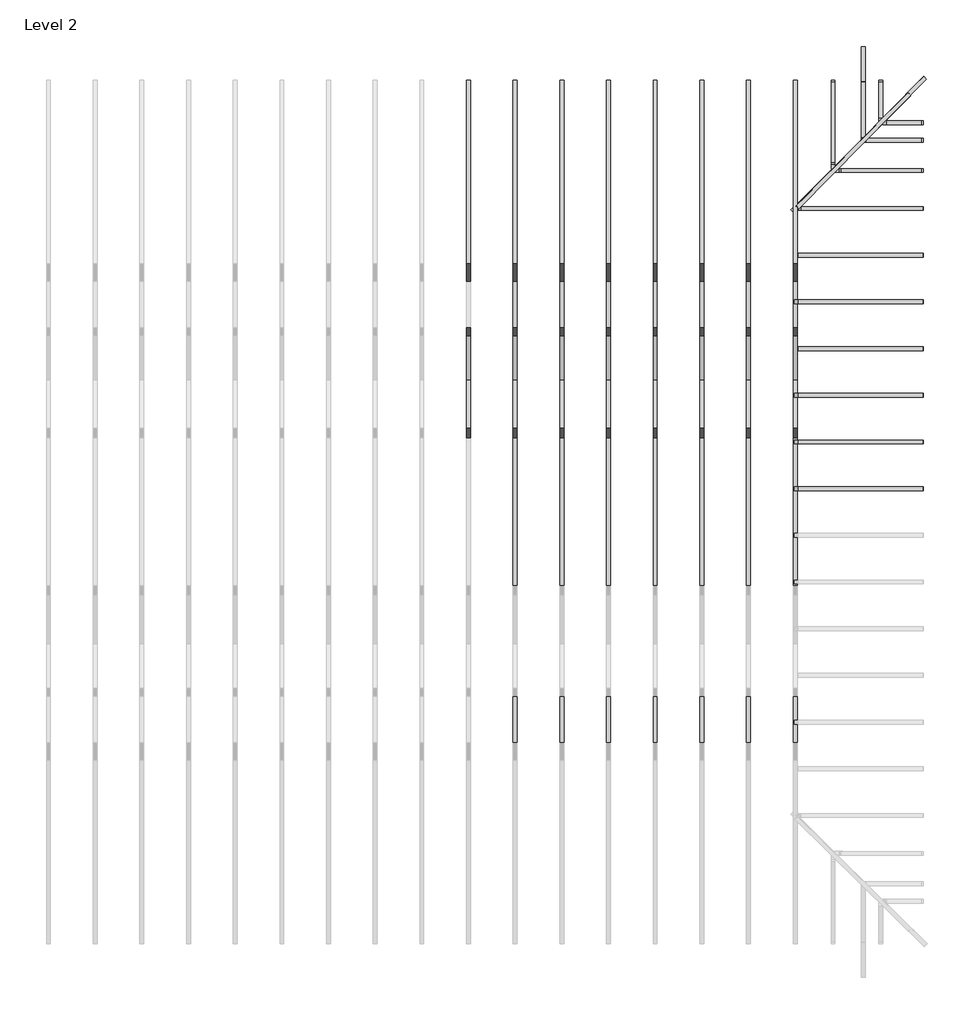
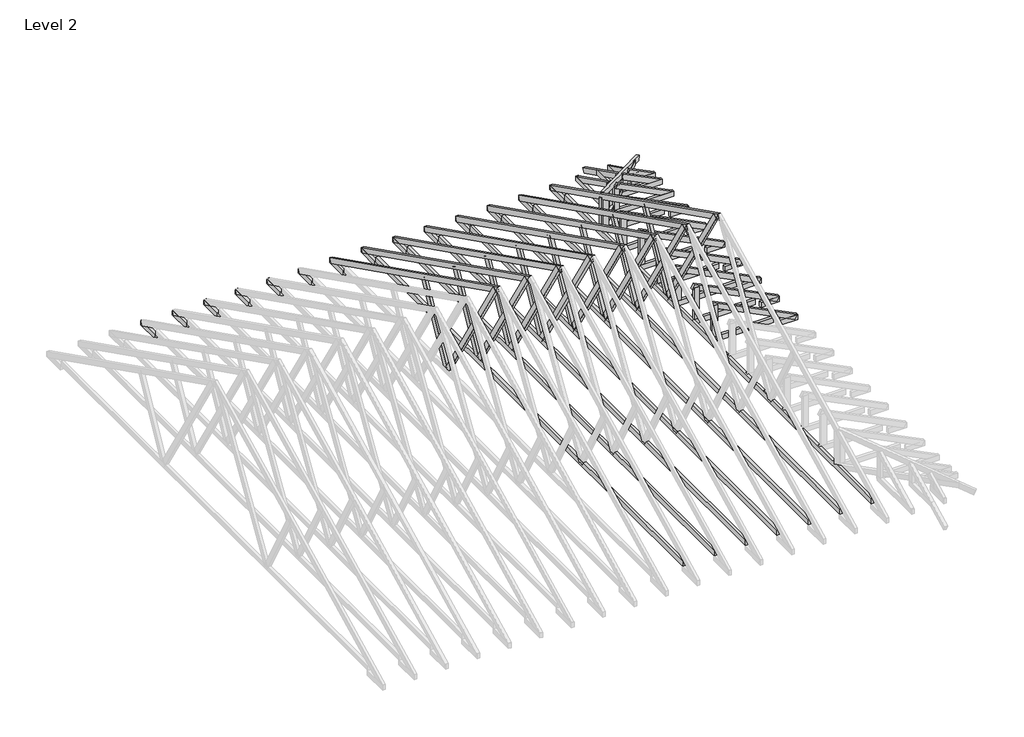
# One storey, part 5 of 5: 94 beams.
"""IFC4 building model written with IfcOpenShell, lengths in millimetres."""

import ifcopenshell
import ifcopenshell.guid

model = None  # the IFC model being written
_history = None  # IfcOwnerHistory: only IFC2X3 demands one
_inside = {}  # id of a spatial element -> (the spatial element, [elements in it])
_under = {}  # id of a project, library or spatial element -> (it, [spatial elements below it])
_declared = {}  # id of a project -> (the project, [libraries it declares])
_typed = {}  # id of a type object -> (the type object, [elements of that type])
_made_of = {}  # id of a material, layer set ... -> (it, [elements and type objects made of it])


def new_model(schema):
    """Start an empty IFC model of exactly this schema.

    Asked for "IFC4X3", IfcOpenShell would pick the latest addendum, in which some entities
    have other attributes; the version numbers below select the first issue.
    IFC2X3 requires an IfcOwnerHistory on every rooted entity: one is made here for all.
    """
    global model, _history
    if schema == "IFC4X3":
        model = ifcopenshell.file(schema_version=(4, 3, 0, 0))
    else:
        model = ifcopenshell.file(schema=schema)
    _inside.clear()
    _under.clear()
    _declared.clear()
    _typed.clear()
    _made_of.clear()
    _history = None
    if model.schema == "IFC2X3":
        org = make("IfcOrganization", Name="unknown")
        user = make(
            "IfcPersonAndOrganization",
            ThePerson=make("IfcPerson", FamilyName="unknown"),
            TheOrganization=org,
        )
        app = make(
            "IfcApplication",
            ApplicationDeveloper=org,
            Version="unknown",
            ApplicationFullName="unknown",
            ApplicationIdentifier="unknown",
        )
        _history = make(
            "IfcOwnerHistory",
            OwningUser=user,
            OwningApplication=app,
            ChangeAction="ADDED",
            CreationDate=0,
        )
    return model


def make(cls, **values):
    """One entity of the class cls with the attributes given. An attribute that is None is left unset."""
    return model.create_entity(
        cls, **{name: value for name, value in values.items() if value is not None}
    )


def rooted(cls, **values):
    """An entity with a GlobalId (a new one), such as an element, a storey or a relation."""
    return make(cls, GlobalId=ifcopenshell.guid.new(), OwnerHistory=_history, **values)


def si_unit(unit_type, name, prefix=None):
    """IfcSIUnit, for example si_unit("LENGTHUNIT", "METRE", prefix="MILLI")."""
    return make("IfcSIUnit", UnitType=unit_type, Prefix=prefix, Name=name)


def assignment(units):
    """IfcUnitAssignment: the units of a project."""
    return None if units is None else make("IfcUnitAssignment", Units=units)


def point(xyz):
    """IfcCartesianPoint."""
    return None if xyz is None else make("IfcCartesianPoint", Coordinates=xyz)


def direction(xyz):
    """IfcDirection."""
    return None if xyz is None else make("IfcDirection", DirectionRatios=xyz)


def frame(location, z_axis=None, x_axis=None):
    """IfcAxis2Placement3D, a coordinate frame: its origin and axes. An axis left out is left unset."""
    return make(
        "IfcAxis2Placement3D",
        Location=point(location),
        Axis=direction(z_axis),
        RefDirection=direction(x_axis),
    )


def origin():
    """The frame at (0, 0, 0) with its axes left unset."""
    return frame((0.0, 0.0, 0.0))


def place(relative_to, where):
    """IfcLocalPlacement: puts the frame where relative to a parent placement (None: the world)."""
    return make(
        "IfcLocalPlacement", PlacementRelTo=relative_to, RelativePlacement=where
    )


def context(
    kind, dimensions, precision=None, world=None, true_north=None, identifier=None
):
    """IfcGeometricRepresentationContext, for example the 3D "Model" context."""
    return make(
        "IfcGeometricRepresentationContext",
        ContextIdentifier=identifier,
        ContextType=kind,
        CoordinateSpaceDimension=dimensions,
        Precision=precision,
        WorldCoordinateSystem=world,
        TrueNorth=true_north,
    )


def project(units=None, contexts=None):
    """IfcProject with its units and contexts."""
    return rooted(
        "IfcProject",
        Name="project",
        RepresentationContexts=contexts,
        UnitsInContext=assignment(units),
    )


def spatial(cls, under=None, at=None, **own):
    """A site, building, storey or space (cls), placed at a placement, below another one or the project."""
    s = rooted(cls, ObjectPlacement=at, **own)
    if under is not None:
        _under.setdefault(under.id(), (under, []))[1].append(s)
    return s


def polyline(points):
    """IfcPolyline through the points."""
    return make("IfcPolyline", Points=[point(p) for p in points])


def outline(outer, holes=None, kind="AREA"):
    """IfcArbitraryClosedProfileDef: a profile drawn as a closed curve; with holes, ...WithVoids."""
    if holes is None:
        return make("IfcArbitraryClosedProfileDef", ProfileType=kind, OuterCurve=outer)
    return make(
        "IfcArbitraryProfileDefWithVoids",
        ProfileType=kind,
        OuterCurve=outer,
        InnerCurves=holes,
    )


def extrude(swept, where, along, depth):
    """IfcExtrudedAreaSolid: the profile swept, set in the frame where, extruded along a direction by depth."""
    return make(
        "IfcExtrudedAreaSolid",
        SweptArea=swept,
        Position=where,
        ExtrudedDirection=direction(along),
        Depth=depth,
    )


def shape(context_of_items, identifier, shape_type, items):
    """IfcShapeRepresentation: the items that make up one representation, for example the "Body"."""
    return make(
        "IfcShapeRepresentation",
        ContextOfItems=context_of_items,
        RepresentationIdentifier=identifier,
        RepresentationType=shape_type,
        Items=items,
    )


def source(mapping_origin, context_of_items, identifier, shape_type, items):
    """IfcRepresentationMap: a shape defined once, which mapped items show again and again."""
    return make(
        "IfcRepresentationMap",
        MappingOrigin=mapping_origin,
        MappedRepresentation=shape(context_of_items, identifier, shape_type, items),
    )


def transform(
    local_origin,
    x_axis=None,
    y_axis=None,
    z_axis=None,
    scale=None,
    scale2=None,
    scale3=None,
    uniform=True,
):
    """IfcCartesianTransformationOperator3D, or its non-uniform kind. x_axis, y_axis, z_axis: its Axis1, 2, 3."""
    if uniform:
        return make(
            "IfcCartesianTransformationOperator3D",
            Axis1=direction(x_axis),
            Axis2=direction(y_axis),
            LocalOrigin=point(local_origin),
            Scale=scale,
            Axis3=direction(z_axis),
        )
    return make(
        "IfcCartesianTransformationOperator3DnonUniform",
        Axis1=direction(x_axis),
        Axis2=direction(y_axis),
        LocalOrigin=point(local_origin),
        Scale=scale,
        Axis3=direction(z_axis),
        Scale2=scale2,
        Scale3=scale3,
    )


def mapped(mapping_source, mapping_target):
    """IfcMappedItem: shows the shape of a source again, moved by a transform."""
    return make(
        "IfcMappedItem", MappingSource=mapping_source, MappingTarget=mapping_target
    )


def made_of(thing, what):
    """Note that an element or type object is made of a material, layer set ...; save() writes the relation."""
    if what is not None:
        _made_of.setdefault(what.id(), (what, []))[1].append(thing)
    return thing


def element(
    cls,
    number,
    at=None,
    inside=None,
    cuts=None,
    type_object=None,
    material=None,
    context=None,
    identifier="Body",
    shape_type=None,
    held_by="IfcProductDefinitionShape",
    body=None,
    shapes=None,
    **own,
):
    """One element of the class cls, such as IfcWall. Its Tag is "e" and its number.

    at: its placement. inside: the storey or other place that contains it. cuts: it is an
    opening in that element (IfcRelVoidsElement). A single representation is given by context,
    identifier, shape_type and body (its items); several are given by shapes. held_by: the class
    of the entity that holds the representations. save() writes the other relations.
    """
    e = rooted(cls, Tag="e%d" % number, ObjectPlacement=at, **own)
    if body is not None:
        shapes = [shape(context, identifier, shape_type, body)]
    if shapes is not None:
        e.Representation = make(held_by, Representations=shapes)
    if inside is not None:
        _inside.setdefault(inside.id(), (inside, []))[1].append(e)
    if cuts is not None:
        rooted(
            "IfcRelVoidsElement", RelatingBuildingElement=cuts, RelatedOpeningElement=e
        )
    if type_object is not None:
        _typed.setdefault(type_object.id(), (type_object, []))[1].append(e)
    return made_of(e, material)


def aggregate(whole, parts):
    """IfcRelAggregates: a whole, such as a stair, and the parts it consists of."""
    return rooted("IfcRelAggregates", RelatingObject=whole, RelatedObjects=parts)


def save(model, path):
    """Write the relations noted so far, then the file.

    IfcRelAggregates (storeys below a building ...), IfcRelContainedInSpatialStructure (elements
    in a storey), IfcRelDefinesByType, IfcRelAssociatesMaterial and IfcRelDeclares: one each for
    every whole, place, type object, material and project.
    """
    for whole, parts in _under.values():
        aggregate(whole, parts)
    for where, things in _inside.values():
        rooted(
            "IfcRelContainedInSpatialStructure",
            RelatedElements=things,
            RelatingStructure=where,
        )
    for kind, things in _typed.values():
        rooted("IfcRelDefinesByType", RelatedObjects=things, RelatingType=kind)
    for what, things in _made_of.values():
        rooted("IfcRelAssociatesMaterial", RelatedObjects=things, RelatingMaterial=what)
    for by, libraries in _declared.values():
        rooted("IfcRelDeclares", RelatingContext=by, RelatedDefinitions=libraries)
    model.write(path)


def beam_b78a0881(model_context):
    return source(origin(), model_context, "Body", "SweptSolid", [
        extrude(outline(polyline([(228.6, 25.4), (228.6, -25.4), (-228.6, -25.4), (-228.6, 25.4), (228.6, 25.4)])), frame((0.0, 0.0, -50.8), z_axis=(0.0, 0.0, 1.0), x_axis=(1.0, 0.0, 0.0)), (0.0, 0.0, 1.0), 101.6),
    ])


def beam_85682148(model_context):
    return source(origin(), model_context, "Body", "SweptSolid", [
        extrude(outline(polyline([(595.8662636, -25.4), (-609.6, -25.4), (-609.6, 25.4), (595.8662636, 25.4), (595.8662636, -25.4)])), frame((0.0, 0.0, -50.8), z_axis=(0.0, 0.0, 1.0), x_axis=(1.0, 0.0, 0.0)), (0.0, 0.0, 1.0), 101.6),
    ])


def beam_f00f3f92(model_context):
    return source(origin(), model_context, "Body", "SweptSolid", [
        extrude(outline(polyline([(393.7, -25.4), (-393.7, -25.4), (-393.7, 25.4), (393.7, 25.4), (393.7, -25.4)])), frame((0.0, 0.0, -50.8), z_axis=(0.0, 0.0, 1.0), x_axis=(1.0, 0.0, 0.0)), (0.0, 0.0, 1.0), 101.6),
    ])


def beam_90eea034(model_context):
    return source(origin(), model_context, "Body", "SweptSolid", [
        extrude(outline(polyline([(821.193698, 25.4), (821.193698, -25.4), (-819.5010489, -25.4), (-819.5010489, 25.4), (821.193698, 25.4)])), frame((0.0, 0.0, -50.8), z_axis=(0.0, 0.0, 1.0), x_axis=(1.0, 0.0, 0.0)), (0.0, 0.0, 1.0), 101.6),
    ])


def beam_a4242642(model_context):
    return source(origin(), model_context, "Body", "SweptSolid", [
        extrude(outline(polyline([(5145.3336481, 25.4), (5145.3336481, -25.4), (-5145.3336481, -25.4), (-5145.3336481, 25.4), (5145.3336481, 25.4)])), frame((0.0, 0.0, -50.8), z_axis=(0.0, 0.0, 1.0), x_axis=(1.0, 0.0, 0.0)), (0.0, 0.0, 1.0), 101.6),
    ])


def beam_fc8bf4ae(model_context):
    return source(origin(), model_context, "Body", "SweptSolid", [
        extrude(outline(polyline([(1562.6646551, 25.4), (1562.6646551, -25.4), (-1550.1468127, -25.4), (-1550.1468127, 25.4), (1562.6646551, 25.4)])), frame((0.0, 0.0, -50.8), z_axis=(0.0, 0.0, 1.0), x_axis=(1.0, 0.0, 0.0)), (0.0, 0.0, 1.0), 101.6),
    ])


def beam_87710fdd(model_context):
    return source(origin(), model_context, "Body", "SweptSolid", [
        extrude(outline(polyline([(147.1272806, 25.4), (147.1272806, -25.4), (-142.875, -25.4), (-142.875, 25.4), (147.1272806, 25.4)])), frame((0.0, 0.0, -50.8), z_axis=(0.0, 0.0, 1.0), x_axis=(1.0, 0.0, 0.0)), (0.0, 0.0, 1.0), 101.6),
    ])


def beam_7b8fa6d1(model_context):
    return source(origin(), model_context, "Body", "SweptSolid", [
        extrude(outline(polyline([(270.7395597, 25.4), (270.7395597, -25.4), (-219.9395597, -25.4), (-219.9395597, 25.4), (270.7395597, 25.4)])), frame((0.0, 0.0, -50.8), z_axis=(0.0, 0.0, 1.0), x_axis=(1.0, 0.0, 0.0)), (0.0, 0.0, 1.0), 101.6),
    ])


def beam_42a29ae5(model_context):
    return source(origin(), model_context, "Body", "SweptSolid", [
        extrude(outline(polyline([(270.7395597, -25.4), (-219.9395597, -25.4), (-219.9395597, 25.4), (270.7395597, 25.4), (270.7395597, -25.4)])), frame((0.0, 0.0, -50.8), z_axis=(0.0, 0.0, 1.0), x_axis=(1.0, 0.0, 0.0)), (0.0, 0.0, 1.0), 101.6),
    ])


def beam_11c5b8ca(model_context):
    return source(origin(), model_context, "Body", "SweptSolid", [
        extrude(outline(polyline([(147.1272806, -25.4), (-142.875, -25.4), (-142.875, 25.4), (147.1272806, 25.4), (147.1272806, -25.4)])), frame((0.0, 0.0, -50.8), z_axis=(0.0, 0.0, 1.0), x_axis=(1.0, 0.0, 0.0)), (0.0, 0.0, 1.0), 101.6),
    ])


def beam_a8bd1fc0(model_context):
    return source(origin(), model_context, "Body", "SweptSolid", [
        extrude(outline(polyline([(571.5, -25.4), (-609.6, -25.4), (-609.6, 25.4), (571.5, 25.4), (571.5, -25.4)])), frame((0.0, 0.0, -50.8), z_axis=(0.0, 0.0, 1.0), x_axis=(1.0, 0.0, 0.0)), (0.0, 0.0, 1.0), 101.6),
    ])


def beam_f5027b49(model_context):
    return source(origin(), model_context, "Body", "SweptSolid", [
        extrude(outline(polyline([(571.5, 25.4), (571.5, -25.4), (-584.2, -25.4), (-584.2, 25.4), (571.5, 25.4)])), frame((0.0, 0.0, -50.8), z_axis=(0.0, 0.0, 1.0), x_axis=(1.0, 0.0, 0.0)), (0.0, 0.0, 1.0), 101.6),
    ])


def beam_78ff79ac(model_context):
    return source(origin(), model_context, "Body", "SweptSolid", [
        extrude(outline(polyline([(365.3019367, -25.4), (-314.5019367, -25.4), (-314.5019367, 25.4), (365.3019367, 25.4), (365.3019367, -25.4)])), frame((0.0, 0.0, -50.8), z_axis=(0.0, 0.0, 1.0), x_axis=(1.0, 0.0, 0.0)), (0.0, 0.0, 1.0), 101.6),
    ])


def beam_99e5442a(model_context):
    return source(origin(), model_context, "Body", "SweptSolid", [
        extrude(outline(polyline([(350.5042173, -25.4), (-295.4519367, -25.4), (-295.4519367, 25.4), (350.5042173, 25.4), (350.5042173, -25.4)])), frame((0.0, 0.0, -50.8), z_axis=(0.0, 0.0, 1.0), x_axis=(1.0, 0.0, 0.0)), (0.0, 0.0, 1.0), 101.6),
    ])


def beam_38e3f9e5(model_context):
    return source(origin(), model_context, "Body", "SweptSolid", [
        extrude(outline(polyline([(595.8662636, -25.4), (-548.2789755, -25.4), (-548.2789755, 25.4), (595.8662636, 25.4), (595.8662636, -25.4)])), frame((0.0, 0.0, -50.8), z_axis=(0.0, 0.0, 1.0), x_axis=(1.0, 0.0, 0.0)), (0.0, 0.0, 1.0), 101.6),
    ])


def beam_7aad778a(model_context):
    return source(origin(), model_context, "Body", "SweptSolid", [
        extrude(outline(polyline([(307.975, -25.4), (-47.625, -25.4), (-47.625, 25.4), (307.975, 25.4), (307.975, -25.4)])), frame((0.0, 0.0, -50.8), z_axis=(0.0, 0.0, 1.0), x_axis=(1.0, 0.0, 0.0)), (0.0, 0.0, 1.0), 101.6),
    ])


def beam_878446a4(model_context):
    return source(origin(), model_context, "Body", "SweptSolid", [
        extrude(outline(polyline([(63.8057136, 25.4), (63.8057136, -25.4), (-59.553433, -25.4), (-59.553433, 25.4), (63.8057136, 25.4)])), frame((0.0, 0.0, -50.8), z_axis=(0.0, 0.0, 1.0), x_axis=(1.0, 0.0, 0.0)), (0.0, 0.0, 1.0), 101.6),
    ])


def beam_bc99fd75(model_context):
    return source(origin(), model_context, "Body", "SweptSolid", [
        extrude(outline(polyline([(222.3387319, 25.4), (222.3387319, -25.4), (-231.775, -25.4), (-231.775, 25.4), (222.3387319, 25.4)])), frame((0.0, 0.0, -50.8), z_axis=(0.0, 0.0, 1.0), x_axis=(1.0, 0.0, 0.0)), (0.0, 0.0, 1.0), 101.6),
    ])


def beam_efe25585(model_context):
    return source(origin(), model_context, "Body", "SweptSolid", [
        extrude(outline(polyline([(222.3387319, -25.4), (-231.775, -25.4), (-231.775, 25.4), (222.3387319, 25.4), (222.3387319, -25.4)])), frame((0.0, 0.0, -50.8), z_axis=(0.0, 0.0, 1.0), x_axis=(1.0, 0.0, 0.0)), (0.0, 0.0, 1.0), 101.6),
    ])


def beam_dfed05dc(model_context):
    return source(origin(), model_context, "Body", "SweptSolid", [
        extrude(outline(polyline([(63.8057136, -25.4), (-59.553433, -25.4), (-59.553433, 25.4), (63.8057136, 25.4), (63.8057136, -25.4)])), frame((0.0, 0.0, -50.8), z_axis=(0.0, 0.0, 1.0), x_axis=(1.0, 0.0, 0.0)), (0.0, 0.0, 1.0), 101.6),
    ])


def beam_0d910f0c(model_context):
    return source(origin(), model_context, "Body", "SweptSolid", [
        extrude(outline(polyline([(233.4866591, -25.4), (-1841.8619641, -25.4), (-1841.8619641, 25.4), (233.4866591, 25.4), (233.4866591, -25.4)])), frame((0.0, 0.0, -50.8), z_axis=(0.0, 0.0, 1.0), x_axis=(1.0, 0.0, 0.0)), (0.0, 0.0, 1.0), 101.6),
    ])


def beam_7b112a02(model_context):
    return source(origin(), model_context, "Body", "SweptSolid", [
        extrude(outline(polyline([(371.7582386, 25.4), (371.7582386, -25.4), (-368.3, -25.4), (-368.3, 25.4), (371.7582386, 25.4)])), frame((0.0, 0.0, -50.8), z_axis=(0.0, 0.0, 1.0), x_axis=(1.0, 0.0, 0.0)), (0.0, 0.0, 1.0), 101.6),
    ])


model = new_model("IFC4")

# Units and contexts
model_context = context("Model", 3, world=origin())
ifc_project = project(units=[si_unit("LENGTHUNIT", "METRE", prefix="MILLI")], contexts=[model_context])

# Site, building, storey
site = spatial("IfcSite", under=ifc_project)
building = spatial("IfcBuilding", under=site)
storey = spatial("IfcBuildingStorey", under=building, Name="Level 2", Elevation=2768.6)

# Beams
placement = place(None, origin())
element("IfcBeam", 1, ObjectType="Dimension Lumber : BLDG 6241 2X4\" TRUSS MEMBER", at=placement, inside=storey, context=model_context, shape_type="SweptSolid", body=[
    extrude(outline(polyline([(0.0, -50.8), (0.0, 0.0), (6302.2496334, 0.0), (6302.2496334, -50.8), (0.0, -50.8)])), frame((-3805.814829, -17.2791662, 5496.1115355), z_axis=(0.0, 0.4472135954999557, 0.894427190999917), x_axis=(0.0, 0.894427190999917, -0.4472135954999557)), (0.0, 0.0, 1.0), 101.6),
])
element("IfcBeam", 2, ObjectType="Dimension Lumber : BLDG 6241 2X4\" TRUSS MEMBER", at=placement, inside=storey, context=model_context, shape_type="SweptSolid", body=[
    extrude(outline(polyline([(0.0, -50.8), (0.0, 0.0), (6302.2496334, 0.0), (6302.2496334, -50.8), (0.0, -50.8)])), frame((-3196.214829, -17.2791662, 5496.1115355), z_axis=(0.0, 0.4472135954999561, 0.8944271909999169), x_axis=(0.0, 0.8944271909999169, -0.4472135954999561)), (0.0, 0.0, 1.0), 101.6),
])
element("IfcBeam", 3, ObjectType="Dimension Lumber : BLDG 6241 2X4\" TRUSS MEMBER", at=placement, inside=storey, context=model_context, shape_type="SweptSolid", body=[
    extrude(outline(polyline([(0.0, -50.8), (0.0, 0.0), (6302.2496334, 0.0), (6302.2496334, -50.8), (0.0, -50.8)])), frame((-2586.614829, -17.2791662, 5496.1115355), z_axis=(0.0, 0.44721359549995593, 0.894427190999917), x_axis=(0.0, 0.894427190999917, -0.44721359549995593)), (0.0, 0.0, 1.0), 101.6),
])
element("IfcBeam", 4, ObjectType="Dimension Lumber : BLDG 6241 2X4\" TRUSS MEMBER", at=placement, inside=storey, context=model_context, shape_type="SweptSolid", body=[
    extrude(outline(polyline([(0.0, -50.8), (0.0, 0.0), (6302.2496334, 0.0), (6302.2496334, -50.8), (0.0, -50.8)])), frame((-1977.014829, -17.2791662, 5496.1115355), z_axis=(0.0, 0.447213595499956, 0.8944271909999169), x_axis=(0.0, 0.8944271909999169, -0.447213595499956)), (0.0, 0.0, 1.0), 101.6),
])
element("IfcBeam", 5, ObjectType="Dimension Lumber : BLDG 6241 2X4\" TRUSS MEMBER", at=placement, inside=storey, context=model_context, shape_type="SweptSolid", body=[
    extrude(outline(polyline([(0.0, -50.8), (0.0, 0.0), (6302.2496334, 0.0), (6302.2496334, -50.8), (0.0, -50.8)])), frame((-1367.414829, -17.2791662, 5496.1115355), z_axis=(0.0, 0.44721359549995593, 0.894427190999917), x_axis=(0.0, 0.894427190999917, -0.44721359549995593)), (0.0, 0.0, 1.0), 101.6),
])
element("IfcBeam", 6, ObjectType="Dimension Lumber : BLDG 6241 2X4\" TRUSS MEMBER", at=placement, inside=storey, context=model_context, shape_type="SweptSolid", body=[
    extrude(outline(polyline([(0.0, -50.8), (0.0, 0.0), (6302.2496334, 0.0), (6302.2496334, -50.8), (0.0, -50.8)])), frame((-757.814829, -17.2791662, 5496.1115355), z_axis=(0.0, 0.4472135954999558, 0.894427190999917), x_axis=(0.0, 0.894427190999917, -0.4472135954999558)), (0.0, 0.0, 1.0), 101.6),
])
element("IfcBeam", 7, ObjectType="Dimension Lumber : BLDG 6241 2X4\" TRUSS MEMBER", at=placement, inside=storey, context=model_context, shape_type="SweptSolid", body=[
    extrude(outline(polyline([(0.0, -50.8), (0.0, 0.0), (6302.2496334, 0.0), (6302.2496334, -50.8), (0.0, -50.8)])), frame((-148.214829, -17.2791662, 5496.1115355), z_axis=(0.0, 0.4472135954999557, 0.894427190999917), x_axis=(0.0, 0.894427190999917, -0.4472135954999557)), (0.0, 0.0, 1.0), 101.6),
])
element("IfcBeam", 8, ObjectType="Dimension Lumber : BLDG 6241 2X4\" TRUSS MEMBER", at=placement, inside=storey, context=model_context, shape_type="SweptSolid", body=[
    extrude(outline(polyline([(0.0, -50.8), (0.0, 0.0), (6302.2496334, 0.0), (6302.2496334, -50.8), (0.0, -50.8)])), frame((461.385171, -17.2791662, 5496.1115355), z_axis=(0.0, 0.4472135954999561, 0.8944271909999169), x_axis=(0.0, 0.8944271909999169, -0.4472135954999561)), (0.0, 0.0, 1.0), 101.6),
])
element("IfcBeam", 9, ObjectType="Dimension Lumber : BLDG 6241 2X4\" TRUSS MEMBER", at=placement, inside=storey, context=model_context, shape_type="SweptSolid", body=[
    extrude(outline(polyline([(0.0, 50.8), (1828.8, 50.8), (1828.8, 0.0), (0.0, 0.0), (0.0, 50.8)])), frame((2110.9853106, 3404.3284114, 2681.1076769), z_axis=(0.44721359549995937, 0.0, 0.8944271909999152), x_axis=(-0.8944271909999152, 0.0, 0.44721359549995937)), (0.0, 0.0, 1.0), 101.6),
])
element("IfcBeam", 10, ObjectType="Dimension Lumber : BLDG 6241 2X4\" TRUSS MEMBER", at=placement, inside=storey, context=model_context, shape_type="SweptSolid", body=[
    extrude(outline(polyline([(0.0, 50.8000001), (2518.7475141, 50.8), (2518.7475141, -1e-07), (0.0, 0.0), (0.0, 50.8000001)])), frame((510.3258967, 3962.9132559, 3515.7397288), z_axis=(0.25320527715849206, 0.22183093198504344, 0.9416358772018716), x_axis=(0.6604274920267093, 0.6716162760239278, -0.33580813801196396)), (0.0, 0.0, 1.0), 101.6),
])
element("IfcBeam", 11, ObjectType="Dimension Lumber : BLDG 6241 2X4\" TRUSS MEMBER", at=placement, inside=storey, context=model_context, shape_type="SweptSolid", body=[
    extrude(outline(polyline([(0.0, 50.8), (1203.6219076, 50.8), (1203.6219076, 0.0), (0.0, 0.0), (0.0, 50.8)])), frame((2112.5153243, 4509.2284114, 2680.3426701), z_axis=(0.44721359549995937, 0.0, 0.8944271909999152), x_axis=(-0.8944271909999152, 0.0, 0.44721359549995937)), (0.0, 0.0, 1.0), 101.6),
])
element("IfcBeam", 12, ObjectType="Dimension Lumber : BLDG 6241 2X4\" TRUSS MEMBER", at=placement, inside=storey, context=model_context, shape_type="SweptSolid", body=[
    extrude(outline(polyline([(0.0, 50.8), (844.55, 50.8), (844.55, 0.0), (0.0, 0.0), (0.0, 50.8)])), frame((2117.2589031, 4902.9284114, 2677.9708807), z_axis=(0.4472135954999599, 0.0, 0.894427190999915), x_axis=(-0.894427190999915, 0.0, 0.4472135954999599)), (0.0, 0.0, 1.0), 101.6),
])
element("IfcBeam", 13, ObjectType="Dimension Lumber : BLDG 6241 2X4\" TRUSS MEMBER", at=placement, inside=storey, context=model_context, shape_type="SweptSolid", body=[
    extrude(outline(polyline([(0.0, 50.8), (1787.5128973, 50.8), (1787.5128973, 0.0), (0.0, 0.0), (0.0, 50.8)])), frame((2110.9853106, 4013.9284114, 2681.1076769), z_axis=(0.44721359549995937, 0.0, 0.8944271909999152), x_axis=(-0.8944271909999152, 0.0, 0.44721359549995937)), (0.0, 0.0, 1.0), 101.6),
])
element("IfcBeam", 14, ObjectType="Dimension Lumber : BLDG 6241 2X4\" TRUSS MEMBER", at=placement, inside=storey, context=model_context, shape_type="SweptSolid", body=[
    extrude(outline(polyline([(0.0, 50.8), (1828.8, 50.8), (1828.8, 0.0), (0.0, 0.0), (0.0, 50.8)])), frame((2110.9853106, 2794.7284114, 2681.1076769), z_axis=(0.44721359549995937, 0.0, 0.8944271909999152), x_axis=(-0.8944271909999152, 0.0, 0.44721359549995937)), (0.0, 0.0, 1.0), 101.6),
])
element("IfcBeam", 15, ObjectType="Dimension Lumber : BLDG 6241 2X4\" TRUSS MEMBER", at=placement, inside=storey, context=model_context, shape_type="SweptSolid", body=[
    extrude(outline(polyline([(0.0, 50.8), (1828.8, 50.8), (1828.8, 0.0), (0.0, 0.0), (0.0, 50.8)])), frame((2110.9853106, 2185.1284114, 2681.1076769), z_axis=(0.44721359549995937, 0.0, 0.8944271909999152), x_axis=(-0.8944271909999152, 0.0, 0.44721359549995937)), (0.0, 0.0, 1.0), 101.6),
])
element("IfcBeam", 16, ObjectType="Dimension Lumber : BLDG 6241 2X4\" TRUSS MEMBER", at=placement, inside=storey, context=model_context, shape_type="SweptSolid", body=[
    extrude(outline(polyline([(0.0, 50.8), (1828.8, 50.8), (1828.8, 0.0), (0.0, 0.0), (0.0, 50.8)])), frame((2110.9853106, 1575.5284114, 2681.1076769), z_axis=(0.44721359549995937, 0.0, 0.8944271909999152), x_axis=(-0.8944271909999152, 0.0, 0.44721359549995937)), (0.0, 0.0, 1.0), 101.6),
])
element("IfcBeam", 17, ObjectType="Dimension Lumber : BLDG 6241 2X4\" TRUSS MEMBER", at=placement, inside=storey, context=model_context, shape_type="SweptSolid", body=[
    extrude(outline(polyline([(0.0, 50.8), (1828.8, 50.8), (1828.8, 0.0), (0.0, 0.0), (0.0, 50.8)])), frame((2110.9853106, 965.9284114, 2681.1076769), z_axis=(0.44721359549995937, 0.0, 0.8944271909999152), x_axis=(-0.8944271909999152, 0.0, 0.44721359549995937)), (0.0, 0.0, 1.0), 101.6),
])
element("IfcBeam", 18, ObjectType="Dimension Lumber : BLDG 6241 2X4\" TRUSS MEMBER", at=placement, inside=storey, context=model_context, shape_type="SweptSolid", body=[
    extrude(outline(polyline([(0.0, 50.8), (1828.8, 50.8), (1828.8, 0.0), (0.0, 0.0), (0.0, 50.8)])), frame((2110.9853106, 356.3284114, 2681.1076769), z_axis=(0.44721359549995937, 0.0, 0.8944271909999152), x_axis=(-0.8944271909999152, 0.0, 0.44721359549995937)), (0.0, 0.0, 1.0), 101.6),
])
element("IfcBeam", 19, ObjectType="Dimension Lumber : BLDG 6241 2X4\" TRUSS MEMBER", at=placement, inside=storey, context=model_context, shape_type="SweptSolid", body=[
    extrude(outline(polyline([(0.0, -50.8), (0.0, 0.0), (1203.6219076, 0.0), (1203.6219076, -50.8), (0.0, -50.8)])), frame((1007.485171, 5614.2585647, 2680.3426701), z_axis=(0.0, 0.44721359549995937, 0.8944271909999152), x_axis=(0.0, -0.8944271909999152, 0.44721359549995937)), (0.0, 0.0, 1.0), 101.6),
])
element("IfcBeam", 20, ObjectType="Dimension Lumber : BLDG 6241 2X4\" TRUSS MEMBER", at=placement, inside=storey, context=model_context, shape_type="SweptSolid", body=[
    extrude(outline(polyline([(0.0, -50.8), (0.0, 0.0), (1334.5727744, 0.0), (1334.5727744, -50.8), (0.0, -50.8)])), frame((1401.185171, 6057.2918371, 2458.8260339), z_axis=(0.0, 0.4472135954999599, 0.894427190999915), x_axis=(0.0, -0.894427190999915, 0.4472135954999599)), (0.0, 0.0, 1.0), 101.6),
])
element("IfcBeam", 21, ObjectType="Dimension Lumber : BLDG 6241 2X4\" TRUSS MEMBER", at=placement, inside=storey, context=model_context, shape_type="SweptSolid", body=[
    extrude(outline(polyline([(0.0, 50.8), (546.1, 50.8), (546.1, 0.0), (0.0, 0.0), (0.0, 50.8)])), frame((2116.9461224, 5131.5284114, 2678.127271), z_axis=(0.4472135954999593, 0.0, 0.8944271909999153), x_axis=(-0.8944271909999153, 0.0, 0.4472135954999593)), (0.0, 0.0, 1.0), 101.6),
])
element("IfcBeam", 22, ObjectType="Dimension Lumber : BLDG 6241 2X4\" TRUSS MEMBER", at=placement, inside=storey, context=model_context, shape_type="SweptSolid", body=[
    extrude(outline(polyline([(0.0, -50.8), (0.0, 0.0), (546.1, 0.0), (546.1, -50.8), (0.0, -50.8)])), frame((1629.785171, 5618.6893628, 2678.127271), z_axis=(0.0, 0.4472135954999592, 0.8944271909999153), x_axis=(0.0, -0.8944271909999153, 0.4472135954999592)), (0.0, 0.0, 1.0), 101.6),
])
beam_shape = beam_b78a0881(model_context)
element("IfcBeam", 23, ObjectType="Dimension Lumber : BLDG 6241 2X4\" TRUSS MEMBER", at=placement, inside=storey, context=model_context, shape_type="MappedRepresentation", body=[
    mapped(beam_shape, transform((-7438.014829, 5436.3284114, 2717.8), x_axis=(0.0, -1.0, 0.0), y_axis=(1.0, 0.0, 0.0), z_axis=(0.0, 0.0, 1.0))),
])
element("IfcBeam", 24, ObjectType="Dimension Lumber : BLDG 6241 2X4\" TRUSS MEMBER", at=placement, inside=storey, context=model_context, shape_type="MappedRepresentation", body=[
    mapped(beam_shape, transform((-6828.414829, 5436.3284114, 2717.8), x_axis=(0.0, -1.0, 0.0), y_axis=(1.0, 0.0, 0.0), z_axis=(0.0, 0.0, 1.0))),
])
element("IfcBeam", 25, ObjectType="Dimension Lumber : BLDG 6241 2X4\" TRUSS MEMBER", at=placement, inside=storey, context=model_context, shape_type="MappedRepresentation", body=[
    mapped(beam_shape, transform((-6218.814829, 5436.3284114, 2717.8), x_axis=(0.0, -1.0, 0.0), y_axis=(1.0, 0.0, 0.0), z_axis=(0.0, 0.0, 1.0))),
])
element("IfcBeam", 26, ObjectType="Dimension Lumber : BLDG 6241 2X4\" TRUSS MEMBER", at=placement, inside=storey, context=model_context, shape_type="MappedRepresentation", body=[
    mapped(beam_shape, transform((-5609.214829, 5436.3284114, 2717.8), x_axis=(0.0, -1.0, 0.0), y_axis=(1.0, 0.0, 0.0), z_axis=(0.0, 0.0, 1.0))),
])
element("IfcBeam", 27, ObjectType="Dimension Lumber : BLDG 6241 2X4\" TRUSS MEMBER", at=placement, inside=storey, context=model_context, shape_type="MappedRepresentation", body=[
    mapped(beam_shape, transform((-4999.614829, 5436.3284114, 2717.8), x_axis=(0.0, -1.0, 0.0), y_axis=(1.0, 0.0, 0.0), z_axis=(0.0, 0.0, 1.0))),
])
element("IfcBeam", 28, ObjectType="Dimension Lumber : BLDG 6241 2X4\" TRUSS MEMBER", at=placement, inside=storey, context=model_context, shape_type="MappedRepresentation", body=[
    mapped(beam_shape, transform((-4390.014829, 5436.3284114, 2717.8), x_axis=(0.0, -1.0, 0.0), y_axis=(1.0, 0.0, 0.0), z_axis=(0.0, 0.0, 1.0))),
])
element("IfcBeam", 29, ObjectType="Dimension Lumber : BLDG 6241 2X4\" TRUSS MEMBER", at=placement, inside=storey, context=model_context, shape_type="MappedRepresentation", body=[
    mapped(beam_shape, transform((-3780.414829, 5436.3284114, 2717.8), x_axis=(0.0, -1.0, 0.0), y_axis=(1.0, 0.0, 0.0), z_axis=(0.0, 0.0, 1.0))),
])
element("IfcBeam", 30, ObjectType="Dimension Lumber : BLDG 6241 2X4\" TRUSS MEMBER", at=placement, inside=storey, context=model_context, shape_type="MappedRepresentation", body=[
    mapped(beam_shape, transform((-3170.814829, 5436.3284114, 2717.8), x_axis=(0.0, -1.0, 0.0), y_axis=(1.0, 0.0, 0.0), z_axis=(0.0, 0.0, 1.0))),
])
element("IfcBeam", 31, ObjectType="Dimension Lumber : BLDG 6241 2X4\" TRUSS MEMBER", at=placement, inside=storey, context=model_context, shape_type="MappedRepresentation", body=[
    mapped(beam_shape, transform((-2561.214829, 5436.3284114, 2717.8), x_axis=(0.0, -1.0, 0.0), y_axis=(1.0, 0.0, 0.0), z_axis=(0.0, 0.0, 1.0))),
])
element("IfcBeam", 32, ObjectType="Dimension Lumber : BLDG 6241 2X4\" TRUSS MEMBER", at=placement, inside=storey, context=model_context, shape_type="MappedRepresentation", body=[
    mapped(beam_shape, transform((-1951.614829, 5436.3284114, 2717.8), x_axis=(0.0, -1.0, 0.0), y_axis=(1.0, 0.0, 0.0), z_axis=(0.0, 0.0, 1.0))),
])
element("IfcBeam", 33, ObjectType="Dimension Lumber : BLDG 6241 2X4\" TRUSS MEMBER", at=placement, inside=storey, context=model_context, shape_type="MappedRepresentation", body=[
    mapped(beam_shape, transform((-1342.014829, 5436.3284114, 2717.8), x_axis=(0.0, -1.0, 0.0), y_axis=(1.0, 0.0, 0.0), z_axis=(0.0, 0.0, 1.0))),
])
element("IfcBeam", 34, ObjectType="Dimension Lumber : BLDG 6241 2X4\" TRUSS MEMBER", at=placement, inside=storey, context=model_context, shape_type="MappedRepresentation", body=[
    mapped(beam_shape, transform((-732.414829, 5436.3284114, 2717.8), x_axis=(0.0, -1.0, 0.0), y_axis=(1.0, 0.0, 0.0), z_axis=(0.0, 0.0, 1.0))),
])
element("IfcBeam", 35, ObjectType="Dimension Lumber : BLDG 6241 2X4\" TRUSS MEMBER", at=placement, inside=storey, context=model_context, shape_type="MappedRepresentation", body=[
    mapped(beam_shape, transform((-122.814829, 5436.3284114, 2717.8), x_axis=(0.0, -1.0, 0.0), y_axis=(1.0, 0.0, 0.0), z_axis=(0.0, 0.0, 1.0))),
])
element("IfcBeam", 36, ObjectType="Dimension Lumber : BLDG 6241 2X4\" TRUSS MEMBER", at=placement, inside=storey, context=model_context, shape_type="MappedRepresentation", body=[
    mapped(beam_shape, transform((486.785171, 5436.3284114, 2717.8), x_axis=(0.0, -1.0, 0.0), y_axis=(1.0, 0.0, 0.0), z_axis=(0.0, 0.0, 1.0))),
])
beam_2_shape = beam_85682148(model_context)
element("IfcBeam", 37, ObjectType="Dimension Lumber : BLDG 6241 2X4\" TRUSS MEMBER", at=placement, inside=storey, context=model_context, shape_type="MappedRepresentation", body=[
    mapped(beam_2_shape, transform((1096.385171, 3378.9284114, 2819.4), x_axis=(1.0, 0.0, 0.0), y_axis=(0.0, 1.0, 0.0), z_axis=(0.0, 0.0, 1.0))),
])
element("IfcBeam", 38, ObjectType="Dimension Lumber : BLDG 6241 2X4\" TRUSS MEMBER", at=placement, inside=storey, context=model_context, shape_type="MappedRepresentation", body=[
    mapped(beam_2_shape, transform((1096.385171, 2769.3284114, 2819.4), x_axis=(1.0, 0.0, 0.0), y_axis=(0.0, 1.0, 0.0), z_axis=(0.0, 0.0, 1.0))),
])
element("IfcBeam", 39, ObjectType="Dimension Lumber : BLDG 6241 2X4\" TRUSS MEMBER", at=placement, inside=storey, context=model_context, shape_type="MappedRepresentation", body=[
    mapped(beam_2_shape, transform((1096.385171, 2159.7284114, 2819.4), x_axis=(1.0, 0.0, 0.0), y_axis=(0.0, 1.0, 0.0), z_axis=(0.0, 0.0, 1.0))),
])
element("IfcBeam", 40, ObjectType="Dimension Lumber : BLDG 6241 2X4\" TRUSS MEMBER", at=placement, inside=storey, context=model_context, shape_type="MappedRepresentation", body=[
    mapped(beam_2_shape, transform((1096.385171, 1550.1284114, 2819.4), x_axis=(1.0, 0.0, 0.0), y_axis=(0.0, 1.0, 0.0), z_axis=(0.0, 0.0, 1.0))),
])
element("IfcBeam", 41, ObjectType="Dimension Lumber : BLDG 6241 2X4\" TRUSS MEMBER", at=placement, inside=storey, context=model_context, shape_type="MappedRepresentation", body=[
    mapped(beam_2_shape, transform((1096.385171, 940.5284114, 2819.4), x_axis=(1.0, 0.0, 0.0), y_axis=(0.0, 1.0, 0.0), z_axis=(0.0, 0.0, 1.0))),
])
element("IfcBeam", 42, ObjectType="Dimension Lumber : BLDG 6241 2X4\" TRUSS MEMBER", at=placement, inside=storey, context=model_context, shape_type="MappedRepresentation", body=[
    mapped(beam_2_shape, transform((1096.385171, 330.9284114, 2819.4), x_axis=(1.0, 0.0, 0.0), y_axis=(0.0, 1.0, 0.0), z_axis=(0.0, 0.0, 1.0))),
])
beam_3_shape = beam_f00f3f92(model_context)
element("IfcBeam", 43, ObjectType="Dimension Lumber : BLDG 6241 2X4\" TRUSS MEMBER", at=placement, inside=storey, context=model_context, shape_type="MappedRepresentation", body=[
    mapped(beam_3_shape, transform((1769.485171, 4877.5284114, 2728.7708807), x_axis=(1.0, 0.0, 0.0), y_axis=(0.0, 1.0, 0.0), z_axis=(0.0, 0.0, 1.0))),
])
beam_4_shape = beam_90eea034(model_context)
element("IfcBeam", 44, ObjectType="Dimension Lumber : BLDG 6241 2X4\" TRUSS MEMBER", at=placement, inside=storey, context=model_context, shape_type="MappedRepresentation", body=[
    mapped(beam_4_shape, transform((-3780.414829, 2147.8781861, 3552.5770493), x_axis=(0.0, -0.4803172630852004, -0.8770948220017847), y_axis=(-1.0, 0.0, 0.0), z_axis=(0.0, 0.8770948220017847, -0.4803172630852004))),
])
element("IfcBeam", 45, ObjectType="Dimension Lumber : BLDG 6241 2X4\" TRUSS MEMBER", at=placement, inside=storey, context=model_context, shape_type="MappedRepresentation", body=[
    mapped(beam_4_shape, transform((-3170.814829, 2147.8781861, 3552.5770493), x_axis=(0.0, -0.4803172630852004, -0.8770948220017847), y_axis=(-1.0, 0.0, 0.0), z_axis=(0.0, 0.8770948220017847, -0.4803172630852004))),
])
element("IfcBeam", 46, ObjectType="Dimension Lumber : BLDG 6241 2X4\" TRUSS MEMBER", at=placement, inside=storey, context=model_context, shape_type="MappedRepresentation", body=[
    mapped(beam_4_shape, transform((-2561.214829, 2147.8781861, 3552.5770493), x_axis=(0.0, -0.4803172630852004, -0.8770948220017847), y_axis=(-1.0, 0.0, 0.0), z_axis=(0.0, 0.8770948220017847, -0.4803172630852004))),
])
element("IfcBeam", 47, ObjectType="Dimension Lumber : BLDG 6241 2X4\" TRUSS MEMBER", at=placement, inside=storey, context=model_context, shape_type="MappedRepresentation", body=[
    mapped(beam_4_shape, transform((-1951.614829, 2147.8781861, 3552.5770493), x_axis=(0.0, -0.4803172630852004, -0.8770948220017847), y_axis=(-1.0, 0.0, 0.0), z_axis=(0.0, 0.8770948220017847, -0.4803172630852004))),
])
element("IfcBeam", 48, ObjectType="Dimension Lumber : BLDG 6241 2X4\" TRUSS MEMBER", at=placement, inside=storey, context=model_context, shape_type="MappedRepresentation", body=[
    mapped(beam_4_shape, transform((-1342.014829, 2147.8781861, 3552.5770493), x_axis=(0.0, -0.4803172630852004, -0.8770948220017847), y_axis=(-1.0, 0.0, 0.0), z_axis=(0.0, 0.8770948220017847, -0.4803172630852004))),
])
element("IfcBeam", 49, ObjectType="Dimension Lumber : BLDG 6241 2X4\" TRUSS MEMBER", at=placement, inside=storey, context=model_context, shape_type="MappedRepresentation", body=[
    mapped(beam_4_shape, transform((-732.414829, 2147.8781861, 3552.5770493), x_axis=(0.0, -0.4803172630852004, -0.8770948220017847), y_axis=(-1.0, 0.0, 0.0), z_axis=(0.0, 0.8770948220017847, -0.4803172630852004))),
])
element("IfcBeam", 50, ObjectType="Dimension Lumber : BLDG 6241 2X4\" TRUSS MEMBER", at=placement, inside=storey, context=model_context, shape_type="MappedRepresentation", body=[
    mapped(beam_4_shape, transform((-122.814829, 2147.8781861, 3552.5770493), x_axis=(0.0, -0.4803172630852004, -0.8770948220017847), y_axis=(-1.0, 0.0, 0.0), z_axis=(0.0, 0.8770948220017847, -0.4803172630852004))),
])
element("IfcBeam", 51, ObjectType="Dimension Lumber : BLDG 6241 2X4\" TRUSS MEMBER", at=placement, inside=storey, context=model_context, shape_type="MappedRepresentation", body=[
    mapped(beam_4_shape, transform((486.785171, 2147.8781861, 3552.5770493), x_axis=(0.0, -0.4803172630852004, -0.8770948220017847), y_axis=(-1.0, 0.0, 0.0), z_axis=(0.0, 0.8770948220017847, -0.4803172630852004))),
])
beam_5_shape = beam_a4242642(model_context)
element("IfcBeam", 52, ObjectType="Dimension Lumber : BLDG 6241 2X4\" TRUSS MEMBER", at=placement, inside=storey, context=model_context, shape_type="MappedRepresentation", body=[
    mapped(beam_5_shape, transform((-3170.814829, 26.1284114, 2819.4), x_axis=(0.0, -1.0, 0.0), y_axis=(1.0, 0.0, 0.0), z_axis=(0.0, 0.0, 1.0))),
])
element("IfcBeam", 53, ObjectType="Dimension Lumber : BLDG 6241 2X4\" TRUSS MEMBER", at=placement, inside=storey, context=model_context, shape_type="MappedRepresentation", body=[
    mapped(beam_5_shape, transform((-2561.214829, 26.1284114, 2819.4), x_axis=(0.0, -1.0, 0.0), y_axis=(1.0, 0.0, 0.0), z_axis=(0.0, 0.0, 1.0))),
])
element("IfcBeam", 54, ObjectType="Dimension Lumber : BLDG 6241 2X4\" TRUSS MEMBER", at=placement, inside=storey, context=model_context, shape_type="MappedRepresentation", body=[
    mapped(beam_5_shape, transform((-1951.614829, 26.1284114, 2819.4), x_axis=(0.0, -1.0, 0.0), y_axis=(1.0, 0.0, 0.0), z_axis=(0.0, 0.0, 1.0))),
])
element("IfcBeam", 55, ObjectType="Dimension Lumber : BLDG 6241 2X4\" TRUSS MEMBER", at=placement, inside=storey, context=model_context, shape_type="MappedRepresentation", body=[
    mapped(beam_5_shape, transform((-1342.014829, 26.1284114, 2819.4), x_axis=(0.0, -1.0, 0.0), y_axis=(1.0, 0.0, 0.0), z_axis=(0.0, 0.0, 1.0))),
])
element("IfcBeam", 56, ObjectType="Dimension Lumber : BLDG 6241 2X4\" TRUSS MEMBER", at=placement, inside=storey, context=model_context, shape_type="MappedRepresentation", body=[
    mapped(beam_5_shape, transform((-732.414829, 26.1284114, 2819.4), x_axis=(0.0, -1.0, 0.0), y_axis=(1.0, 0.0, 0.0), z_axis=(0.0, 0.0, 1.0))),
])
element("IfcBeam", 57, ObjectType="Dimension Lumber : BLDG 6241 2X4\" TRUSS MEMBER", at=placement, inside=storey, context=model_context, shape_type="MappedRepresentation", body=[
    mapped(beam_5_shape, transform((-122.814829, 26.1284114, 2819.4), x_axis=(0.0, -1.0, 0.0), y_axis=(1.0, 0.0, 0.0), z_axis=(0.0, 0.0, 1.0))),
])
element("IfcBeam", 58, ObjectType="Dimension Lumber : BLDG 6241 2X4\" TRUSS MEMBER", at=placement, inside=storey, context=model_context, shape_type="MappedRepresentation", body=[
    mapped(beam_5_shape, transform((486.785171, 26.1284114, 2819.4), x_axis=(0.0, -1.0, 0.0), y_axis=(1.0, 0.0, 0.0), z_axis=(0.0, 0.0, 1.0))),
])
beam_6_shape = beam_fc8bf4ae(model_context)
element("IfcBeam", 59, ObjectType="Dimension Lumber : BLDG 6241 2X4\" TRUSS MEMBER", at=placement, inside=storey, context=model_context, shape_type="MappedRepresentation", body=[
    mapped(beam_6_shape, transform((-3780.414829, 944.3448606, 4154.3437121), x_axis=(0.0, -0.5218941539815979, 0.8530102531856415), y_axis=(-1.0, 0.0, 0.0), z_axis=(0.0, -0.8530102531856415, -0.5218941539815979))),
])
element("IfcBeam", 60, ObjectType="Dimension Lumber : BLDG 6241 2X4\" TRUSS MEMBER", at=placement, inside=storey, context=model_context, shape_type="MappedRepresentation", body=[
    mapped(beam_6_shape, transform((-3170.814829, 944.3448606, 4154.3437121), x_axis=(0.0, -0.5218941539815979, 0.8530102531856415), y_axis=(-1.0, 0.0, 0.0), z_axis=(0.0, -0.8530102531856415, -0.5218941539815979))),
])
element("IfcBeam", 61, ObjectType="Dimension Lumber : BLDG 6241 2X4\" TRUSS MEMBER", at=placement, inside=storey, context=model_context, shape_type="MappedRepresentation", body=[
    mapped(beam_6_shape, transform((-2561.214829, 944.3448606, 4154.3437121), x_axis=(0.0, -0.5218941539815979, 0.8530102531856415), y_axis=(-1.0, 0.0, 0.0), z_axis=(0.0, -0.8530102531856415, -0.5218941539815979))),
])
element("IfcBeam", 62, ObjectType="Dimension Lumber : BLDG 6241 2X4\" TRUSS MEMBER", at=placement, inside=storey, context=model_context, shape_type="MappedRepresentation", body=[
    mapped(beam_6_shape, transform((-1951.614829, 944.3448606, 4154.3437121), x_axis=(0.0, -0.5218941539815979, 0.8530102531856415), y_axis=(-1.0, 0.0, 0.0), z_axis=(0.0, -0.8530102531856415, -0.5218941539815979))),
])
element("IfcBeam", 63, ObjectType="Dimension Lumber : BLDG 6241 2X4\" TRUSS MEMBER", at=placement, inside=storey, context=model_context, shape_type="MappedRepresentation", body=[
    mapped(beam_6_shape, transform((-1342.014829, 944.3448606, 4154.3437121), x_axis=(0.0, -0.5218941539815979, 0.8530102531856415), y_axis=(-1.0, 0.0, 0.0), z_axis=(0.0, -0.8530102531856415, -0.5218941539815979))),
])
element("IfcBeam", 64, ObjectType="Dimension Lumber : BLDG 6241 2X4\" TRUSS MEMBER", at=placement, inside=storey, context=model_context, shape_type="MappedRepresentation", body=[
    mapped(beam_6_shape, transform((-732.414829, 944.3448606, 4154.3437121), x_axis=(0.0, -0.5218941539815979, 0.8530102531856415), y_axis=(-1.0, 0.0, 0.0), z_axis=(0.0, -0.8530102531856415, -0.5218941539815979))),
])
element("IfcBeam", 65, ObjectType="Dimension Lumber : BLDG 6241 2X4\" TRUSS MEMBER", at=placement, inside=storey, context=model_context, shape_type="MappedRepresentation", body=[
    mapped(beam_6_shape, transform((-122.814829, 944.3448606, 4154.3437121), x_axis=(0.0, -0.5218941539815979, 0.8530102531856415), y_axis=(-1.0, 0.0, 0.0), z_axis=(0.0, -0.8530102531856415, -0.5218941539815979))),
])
element("IfcBeam", 66, ObjectType="Dimension Lumber : BLDG 6241 2X4\" TRUSS MEMBER", at=placement, inside=storey, context=model_context, shape_type="MappedRepresentation", body=[
    mapped(beam_6_shape, transform((486.785171, 944.3448606, 4154.3437121), x_axis=(0.0, -0.5218941539815979, 0.8530102531856415), y_axis=(-1.0, 0.0, 0.0), z_axis=(0.0, -0.8530102531856415, -0.5218941539815979))),
])
beam_7_shape = beam_87710fdd(model_context)
element("IfcBeam", 67, ObjectType="Dimension Lumber : BLDG 6241 2X4\" TRUSS MEMBER", at=placement, inside=storey, context=model_context, shape_type="MappedRepresentation", body=[
    mapped(beam_7_shape, transform((1375.785171, 4953.7284114, 2924.5288734), x_axis=(0.0, 0.0, 1.0), y_axis=(1.0, 0.0, 0.0), z_axis=(0.0, 1.0, 0.0))),
])
beam_8_shape = beam_7b8fa6d1(model_context)
element("IfcBeam", 68, ObjectType="Dimension Lumber : BLDG 6241 2X4\" TRUSS MEMBER", at=placement, inside=storey, context=model_context, shape_type="MappedRepresentation", body=[
    mapped(beam_8_shape, transform((982.085171, 4560.0284114, 2999.5104403), x_axis=(0.0, 0.0, 1.0), y_axis=(1.0, 0.0, 0.0), z_axis=(0.0, 1.0, 0.0))),
])
beam_9_shape = beam_42a29ae5(model_context)
element("IfcBeam", 69, ObjectType="Dimension Lumber : BLDG 6241 2X4\" TRUSS MEMBER", at=placement, inside=storey, context=model_context, shape_type="MappedRepresentation", body=[
    mapped(beam_9_shape, transform((1058.285171, 4483.8284114, 2999.5104403), x_axis=(0.0, 0.0, 1.0), y_axis=(0.0, -1.0, 0.0), z_axis=(1.0, 0.0, 0.0))),
])
beam_10_shape = beam_11c5b8ca(model_context)
element("IfcBeam", 70, ObjectType="Dimension Lumber : BLDG 6241 2X4\" TRUSS MEMBER", at=placement, inside=storey, context=model_context, shape_type="MappedRepresentation", body=[
    mapped(beam_10_shape, transform((1451.985171, 4877.5284114, 2924.5288734), x_axis=(0.0, 0.0, 1.0), y_axis=(0.0, -1.0, 0.0), z_axis=(1.0, 0.0, 0.0))),
])
beam_11_shape = beam_a8bd1fc0(model_context)
element("IfcBeam", 71, ObjectType="Dimension Lumber : BLDG 6241 2X4\" TRUSS MEMBER", at=placement, inside=storey, context=model_context, shape_type="MappedRepresentation", body=[
    mapped(beam_11_shape, transform((1591.685171, 4483.8284114, 2728.7708807), x_axis=(1.0, 0.0, 0.0), y_axis=(0.0, 1.0, 0.0), z_axis=(0.0, 0.0, 1.0))),
])
beam_12_shape = beam_f5027b49(model_context)
element("IfcBeam", 72, ObjectType="Dimension Lumber : BLDG 6241 2X4\" TRUSS MEMBER", at=placement, inside=storey, context=model_context, shape_type="MappedRepresentation", body=[
    mapped(beam_12_shape, transform((982.085171, 5093.4284114, 2728.7708807), x_axis=(0.0, 1.0, 0.0), y_axis=(-1.0, 0.0, 0.0), z_axis=(0.0, 0.0, 1.0))),
])
beam_13_shape = beam_78ff79ac(model_context)
element("IfcBeam", 73, ObjectType="Dimension Lumber : BLDG 6241 2X4\" TRUSS MEMBER", at=placement, inside=storey, context=model_context, shape_type="MappedRepresentation", body=[
    mapped(beam_13_shape, transform((486.785171, 3988.5284114, 3184.7019367), x_axis=(0.0, 0.0, 1.0), y_axis=(-0.7071067811865477, 0.7071067811865474, 0.0), z_axis=(-0.7071067811865474, -0.7071067811865477, 0.0))),
])
beam_14_shape = beam_99e5442a(model_context)
element("IfcBeam", 74, ObjectType="Dimension Lumber : BLDG 6241 2X4\" TRUSS MEMBER", at=placement, inside=storey, context=model_context, shape_type="MappedRepresentation", body=[
    mapped(beam_14_shape, transform((562.985171, 3378.9284114, 3165.6519367), x_axis=(0.0, 0.0, 1.0), y_axis=(0.0, -1.0, 0.0), z_axis=(1.0, 0.0, 0.0))),
])
element("IfcBeam", 75, ObjectType="Dimension Lumber : BLDG 6241 2X4\" TRUSS MEMBER", at=placement, inside=storey, context=model_context, shape_type="MappedRepresentation", body=[
    mapped(beam_14_shape, transform((562.985171, 3988.5284114, 3165.6519367), x_axis=(0.0, 0.0, 1.0), y_axis=(0.0, -1.0, 0.0), z_axis=(1.0, 0.0, 0.0))),
])
element("IfcBeam", 76, ObjectType="Dimension Lumber : BLDG 6241 2X4\" TRUSS MEMBER", at=placement, inside=storey, context=model_context, shape_type="MappedRepresentation", body=[
    mapped(beam_14_shape, transform((562.985171, 2769.3284114, 3165.6519367), x_axis=(0.0, 0.0, 1.0), y_axis=(0.0, -1.0, 0.0), z_axis=(1.0, 0.0, 0.0))),
])
element("IfcBeam", 77, ObjectType="Dimension Lumber : BLDG 6241 2X4\" TRUSS MEMBER", at=placement, inside=storey, context=model_context, shape_type="MappedRepresentation", body=[
    mapped(beam_14_shape, transform((562.985171, 2159.7284114, 3165.6519367), x_axis=(0.0, 0.0, 1.0), y_axis=(0.0, -1.0, 0.0), z_axis=(1.0, 0.0, 0.0))),
])
element("IfcBeam", 78, ObjectType="Dimension Lumber : BLDG 6241 2X4\" TRUSS MEMBER", at=placement, inside=storey, context=model_context, shape_type="MappedRepresentation", body=[
    mapped(beam_14_shape, transform((562.985171, 1550.1284114, 3165.6519367), x_axis=(0.0, 0.0, 1.0), y_axis=(0.0, -1.0, 0.0), z_axis=(1.0, 0.0, 0.0))),
])
element("IfcBeam", 79, ObjectType="Dimension Lumber : BLDG 6241 2X4\" TRUSS MEMBER", at=placement, inside=storey, context=model_context, shape_type="MappedRepresentation", body=[
    mapped(beam_14_shape, transform((562.985171, 940.5284114, 3165.6519367), x_axis=(0.0, 0.0, 1.0), y_axis=(0.0, -1.0, 0.0), z_axis=(1.0, 0.0, 0.0))),
])
element("IfcBeam", 80, ObjectType="Dimension Lumber : BLDG 6241 2X4\" TRUSS MEMBER", at=placement, inside=storey, context=model_context, shape_type="MappedRepresentation", body=[
    mapped(beam_14_shape, transform((562.985171, 330.9284114, 3165.6519367), x_axis=(0.0, 0.0, 1.0), y_axis=(0.0, -1.0, 0.0), z_axis=(1.0, 0.0, 0.0))),
])
beam_15_shape = beam_38e3f9e5(model_context)
element("IfcBeam", 81, ObjectType="Dimension Lumber : BLDG 6241 2X4\" TRUSS MEMBER", at=placement, inside=storey, context=model_context, shape_type="MappedRepresentation", body=[
    mapped(beam_15_shape, transform((1096.385171, 3988.5284114, 2819.4), x_axis=(1.0, 0.0, 0.0), y_axis=(0.0, 1.0, 0.0), z_axis=(0.0, 0.0, 1.0))),
])
beam_16_shape = beam_7aad778a(model_context)
element("IfcBeam", 82, ObjectType="Dimension Lumber : BLDG 6241 2X4\" TRUSS MEMBER", at=placement, inside=storey, context=model_context, shape_type="MappedRepresentation", body=[
    mapped(beam_16_shape, transform((2115.560171, 3378.9284114, 2717.8), x_axis=(-1.0, 0.0, 0.0), y_axis=(0.0, -1.0, 0.0), z_axis=(0.0, 0.0, 1.0))),
])
element("IfcBeam", 83, ObjectType="Dimension Lumber : BLDG 6241 2X4\" TRUSS MEMBER", at=placement, inside=storey, context=model_context, shape_type="MappedRepresentation", body=[
    mapped(beam_16_shape, transform((2115.560171, 3988.5284114, 2717.8), x_axis=(-1.0, 0.0, 0.0), y_axis=(0.0, -1.0, 0.0), z_axis=(0.0, 0.0, 1.0))),
])
element("IfcBeam", 84, ObjectType="Dimension Lumber : BLDG 6241 2X4\" TRUSS MEMBER", at=placement, inside=storey, context=model_context, shape_type="MappedRepresentation", body=[
    mapped(beam_16_shape, transform((2115.560171, 2769.3284114, 2717.8), x_axis=(-1.0, 0.0, 0.0), y_axis=(0.0, -1.0, 0.0), z_axis=(0.0, 0.0, 1.0))),
])
element("IfcBeam", 85, ObjectType="Dimension Lumber : BLDG 6241 2X4\" TRUSS MEMBER", at=placement, inside=storey, context=model_context, shape_type="MappedRepresentation", body=[
    mapped(beam_16_shape, transform((2115.560171, 2159.7284114, 2717.8), x_axis=(-1.0, 0.0, 0.0), y_axis=(0.0, -1.0, 0.0), z_axis=(0.0, 0.0, 1.0))),
])
element("IfcBeam", 86, ObjectType="Dimension Lumber : BLDG 6241 2X4\" TRUSS MEMBER", at=placement, inside=storey, context=model_context, shape_type="MappedRepresentation", body=[
    mapped(beam_16_shape, transform((2115.560171, 1550.1284114, 2717.8), x_axis=(-1.0, 0.0, 0.0), y_axis=(0.0, -1.0, 0.0), z_axis=(0.0, 0.0, 1.0))),
])
element("IfcBeam", 87, ObjectType="Dimension Lumber : BLDG 6241 2X4\" TRUSS MEMBER", at=placement, inside=storey, context=model_context, shape_type="MappedRepresentation", body=[
    mapped(beam_16_shape, transform((2115.560171, 940.5284114, 2717.8), x_axis=(-1.0, 0.0, 0.0), y_axis=(0.0, -1.0, 0.0), z_axis=(0.0, 0.0, 1.0))),
])
element("IfcBeam", 88, ObjectType="Dimension Lumber : BLDG 6241 2X4\" TRUSS MEMBER", at=placement, inside=storey, context=model_context, shape_type="MappedRepresentation", body=[
    mapped(beam_16_shape, transform((2115.560171, 330.9284114, 2717.8), x_axis=(-1.0, 0.0, 0.0), y_axis=(0.0, -1.0, 0.0), z_axis=(0.0, 0.0, 1.0))),
])
beam_17_shape = beam_878446a4(model_context)
element("IfcBeam", 89, ObjectType="Dimension Lumber : BLDG 6241 2X4\" TRUSS MEMBER", at=placement, inside=storey, context=model_context, shape_type="MappedRepresentation", body=[
    mapped(beam_17_shape, transform((1604.385171, 5287.0146794, 2841.2073064), x_axis=(0.0, 0.0, 1.0), y_axis=(1.0, 0.0, 0.0), z_axis=(0.0, 1.0, 0.0))),
])
beam_18_shape = beam_bc99fd75(model_context)
element("IfcBeam", 90, ObjectType="Dimension Lumber : BLDG 6241 2X4\" TRUSS MEMBER", at=placement, inside=storey, context=model_context, shape_type="MappedRepresentation", body=[
    mapped(beam_18_shape, transform((1604.385171, 5442.5896794, 2728.7708807), x_axis=(0.0, 1.0, 0.0), y_axis=(-1.0, 0.0, 0.0), z_axis=(0.0, 0.0, 1.0))),
])
beam_19_shape = beam_efe25585(model_context)
element("IfcBeam", 91, ObjectType="Dimension Lumber : BLDG 6241 2X4\" TRUSS MEMBER", at=placement, inside=storey, context=model_context, shape_type="MappedRepresentation", body=[
    mapped(beam_19_shape, transform((1940.846439, 5106.1284114, 2728.7708807), x_axis=(1.0, 0.0, 0.0), y_axis=(0.0, 1.0, 0.0), z_axis=(0.0, 0.0, 1.0))),
])
beam_20_shape = beam_dfed05dc(model_context)
element("IfcBeam", 92, ObjectType="Dimension Lumber : BLDG 6241 2X4\" TRUSS MEMBER", at=placement, inside=storey, context=model_context, shape_type="MappedRepresentation", body=[
    mapped(beam_20_shape, transform((1785.271439, 5106.1284114, 2841.2073064), x_axis=(0.0, 0.0, 1.0), y_axis=(0.0, -1.0, 0.0), z_axis=(1.0, 0.0, 0.0))),
])
beam_21_shape = beam_0d910f0c(model_context)
element("IfcBeam", 93, ObjectType="Dimension Lumber : BLDG 6241 2X4\" TRUSS MEMBER", at=placement, inside=storey, context=model_context, shape_type="MappedRepresentation", body=[
    mapped(beam_21_shape, transform((677.285171, 4179.0284114, 2819.4), x_axis=(-0.7071067811865462, -0.7071067811865488, 0.0), y_axis=(0.7071067811865488, -0.7071067811865462, 0.0), z_axis=(0.0, 0.0, 1.0))),
])
beam_22_shape = beam_7b112a02(model_context)
element("IfcBeam", 94, ObjectType="Dimension Lumber : BLDG 6241 2X4\" TRUSS MEMBER", at=placement, inside=storey, context=model_context, shape_type="MappedRepresentation", body=[
    mapped(beam_22_shape, transform((1375.785171, 5271.2284114, 2728.7708807), x_axis=(0.0, 1.0, 0.0), y_axis=(-1.0, 0.0, 0.0), z_axis=(0.0, 0.0, 1.0))),
])

save(model, "model.ifc")

# Revit data of these elements
# Type "Dimension Lumber : BLDG 6241 2X4\" TRUSS MEMBER"
#   Assembly Code = "B10"
#   A = 0.273472 SF
#   Length [instance default] = 5' - 0"
#   b = 0' - 2"
#   d = 0' - 4"
#   Structural Material [instance default] = Softwood, Lumber
# Elements 1, 2, 3, 4, 5, 6, 7, 8, 9, 10, 11, 12, 13, 14, 15, 16, 17, 18, 19, 20, 21, 22, 37, 38, 39, 40, 41, 42, 43, 44, 45, 46, 47, 48, 49, 50, 51, 52, 53, 54, 55, 56, 57, 58, 59, 60, 61, 62, 63, 64, 65, 66, 67, 68, 69, 70, 71, 72, 73, 74, 75, 76, 77, 78, 79, 80, 81, 89, 90, 91, 92, 93, 94 (IfcBeam, "Dimension Lumber : BLDG 6241 2X4\" TRUSS MEMBER")
#   Structural Material = Softwood, Lumber
#   Phase Created = New Construction
#   Materials on its faces: "Softwood, Lumber"
# Elements 23, 24, 25, 26, 27, 28, 29, 30, 31, 32, 33, 34, 35, 36, 82, 83, 84, 85, 86, 87, 88 (IfcBeam, "Dimension Lumber : BLDG 6241 2X4\" TRUSS MEMBER")
#   Comments = ""
#   Structural Material = Softwood, Lumber
#   Phase Created = New Construction
#   Materials on its faces: "Softwood, Lumber"
# Materials
#   "Softwood, Lumber": class "Wood", colour RGB 223 192 134, transparency 0, Description = "Pinus Echinata", Cost = 0
